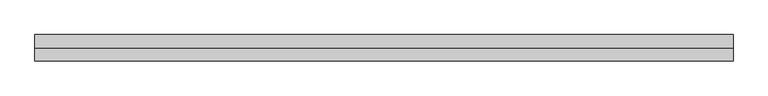
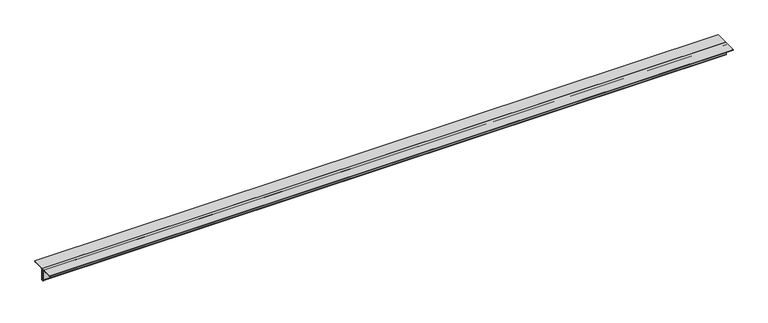
"""IFC4 building model written with IfcOpenShell, lengths in millimetres: member geometry, 0123_Steel Framing_2Ls-KSD3502 : H_SB_AR_S03_2Ls-130x130x12_HBR4."""

import ifcopenshell
import ifcopenshell.guid

model = None  # the IFC model being written
_history = None  # IfcOwnerHistory: only IFC2X3 demands one
_inside = {}  # id of a spatial element -> (the spatial element, [elements in it])
_under = {}  # id of a project, library or spatial element -> (it, [spatial elements below it])
_declared = {}  # id of a project -> (the project, [libraries it declares])
_typed = {}  # id of a type object -> (the type object, [elements of that type])
_made_of = {}  # id of a material, layer set ... -> (it, [elements and type objects made of it])


def new_model(schema):
    """Start an empty IFC model of exactly this schema.

    Asked for "IFC4X3", IfcOpenShell would pick the latest addendum, in which some entities
    have other attributes; the version numbers below select the first issue.
    IFC2X3 requires an IfcOwnerHistory on every rooted entity: one is made here for all.
    """
    global model, _history
    if schema == "IFC4X3":
        model = ifcopenshell.file(schema_version=(4, 3, 0, 0))
    else:
        model = ifcopenshell.file(schema=schema)
    _inside.clear()
    _under.clear()
    _declared.clear()
    _typed.clear()
    _made_of.clear()
    _history = None
    if model.schema == "IFC2X3":
        org = make("IfcOrganization", Name="unknown")
        user = make(
            "IfcPersonAndOrganization",
            ThePerson=make("IfcPerson", FamilyName="unknown"),
            TheOrganization=org,
        )
        app = make(
            "IfcApplication",
            ApplicationDeveloper=org,
            Version="unknown",
            ApplicationFullName="unknown",
            ApplicationIdentifier="unknown",
        )
        _history = make(
            "IfcOwnerHistory",
            OwningUser=user,
            OwningApplication=app,
            ChangeAction="ADDED",
            CreationDate=0,
        )
    return model


def make(cls, **values):
    """One entity of the class cls with the attributes given. An attribute that is None is left unset."""
    return model.create_entity(
        cls, **{name: value for name, value in values.items() if value is not None}
    )


def rooted(cls, **values):
    """An entity with a GlobalId (a new one), such as an element, a storey or a relation."""
    return make(cls, GlobalId=ifcopenshell.guid.new(), OwnerHistory=_history, **values)


def si_unit(unit_type, name, prefix=None):
    """IfcSIUnit, for example si_unit("LENGTHUNIT", "METRE", prefix="MILLI")."""
    return make("IfcSIUnit", UnitType=unit_type, Prefix=prefix, Name=name)


def assignment(units):
    """IfcUnitAssignment: the units of a project."""
    return None if units is None else make("IfcUnitAssignment", Units=units)


def point(xyz):
    """IfcCartesianPoint."""
    return None if xyz is None else make("IfcCartesianPoint", Coordinates=xyz)


def direction(xyz):
    """IfcDirection."""
    return None if xyz is None else make("IfcDirection", DirectionRatios=xyz)


def frame(location, z_axis=None, x_axis=None):
    """IfcAxis2Placement3D, a coordinate frame: its origin and axes. An axis left out is left unset."""
    return make(
        "IfcAxis2Placement3D",
        Location=point(location),
        Axis=direction(z_axis),
        RefDirection=direction(x_axis),
    )


def frame_2d(location, x_axis=None):
    """IfcAxis2Placement2D, a coordinate frame in the plane: its origin and x axis."""
    return make(
        "IfcAxis2Placement2D", Location=point(location), RefDirection=direction(x_axis)
    )


def origin():
    """The frame at (0, 0, 0) with its axes left unset."""
    return frame((0.0, 0.0, 0.0))


def place(relative_to, where):
    """IfcLocalPlacement: puts the frame where relative to a parent placement (None: the world)."""
    return make(
        "IfcLocalPlacement", PlacementRelTo=relative_to, RelativePlacement=where
    )


def context(
    kind, dimensions, precision=None, world=None, true_north=None, identifier=None
):
    """IfcGeometricRepresentationContext, for example the 3D "Model" context."""
    return make(
        "IfcGeometricRepresentationContext",
        ContextIdentifier=identifier,
        ContextType=kind,
        CoordinateSpaceDimension=dimensions,
        Precision=precision,
        WorldCoordinateSystem=world,
        TrueNorth=true_north,
    )


def project(units=None, contexts=None):
    """IfcProject with its units and contexts."""
    return rooted(
        "IfcProject",
        Name="project",
        RepresentationContexts=contexts,
        UnitsInContext=assignment(units),
    )


def spatial(cls, under=None, at=None, **own):
    """A site, building, storey or space (cls), placed at a placement, below another one or the project."""
    s = rooted(cls, ObjectPlacement=at, **own)
    if under is not None:
        _under.setdefault(under.id(), (under, []))[1].append(s)
    return s


def polyline(points):
    """IfcPolyline through the points."""
    return make("IfcPolyline", Points=[point(p) for p in points])


def circle_curve(where, radius):
    """IfcCircle in the frame where."""
    return make("IfcCircle", Position=where, Radius=radius)


def trimmed(basis, trim1, trim2, sense, master):
    """IfcTrimmedCurve: the piece of a basis curve between two trims."""
    return make(
        "IfcTrimmedCurve",
        BasisCurve=basis,
        Trim1=trim1,
        Trim2=trim2,
        SenseAgreement=sense,
        MasterRepresentation=master,
    )


def segment(curve, same_sense, transition):
    """IfcCompositeCurveSegment."""
    return make(
        "IfcCompositeCurveSegment",
        Transition=transition,
        SameSense=same_sense,
        ParentCurve=curve,
    )


def composite_curve(segments, self_intersect=None):
    """IfcCompositeCurve: segments joined end to end."""
    return make("IfcCompositeCurve", Segments=segments, SelfIntersect=self_intersect)


def outline(outer, holes=None, kind="AREA"):
    """IfcArbitraryClosedProfileDef: a profile drawn as a closed curve; with holes, ...WithVoids."""
    if holes is None:
        return make("IfcArbitraryClosedProfileDef", ProfileType=kind, OuterCurve=outer)
    return make(
        "IfcArbitraryProfileDefWithVoids",
        ProfileType=kind,
        OuterCurve=outer,
        InnerCurves=holes,
    )


def extrude(swept, where, along, depth):
    """IfcExtrudedAreaSolid: the profile swept, set in the frame where, extruded along a direction by depth."""
    return make(
        "IfcExtrudedAreaSolid",
        SweptArea=swept,
        Position=where,
        ExtrudedDirection=direction(along),
        Depth=depth,
    )


def shape(context_of_items, identifier, shape_type, items):
    """IfcShapeRepresentation: the items that make up one representation, for example the "Body"."""
    return make(
        "IfcShapeRepresentation",
        ContextOfItems=context_of_items,
        RepresentationIdentifier=identifier,
        RepresentationType=shape_type,
        Items=items,
    )


def source(mapping_origin, context_of_items, identifier, shape_type, items):
    """IfcRepresentationMap: a shape defined once, which mapped items show again and again."""
    return make(
        "IfcRepresentationMap",
        MappingOrigin=mapping_origin,
        MappedRepresentation=shape(context_of_items, identifier, shape_type, items),
    )


def transform(
    local_origin,
    x_axis=None,
    y_axis=None,
    z_axis=None,
    scale=None,
    scale2=None,
    scale3=None,
    uniform=True,
):
    """IfcCartesianTransformationOperator3D, or its non-uniform kind. x_axis, y_axis, z_axis: its Axis1, 2, 3."""
    if uniform:
        return make(
            "IfcCartesianTransformationOperator3D",
            Axis1=direction(x_axis),
            Axis2=direction(y_axis),
            LocalOrigin=point(local_origin),
            Scale=scale,
            Axis3=direction(z_axis),
        )
    return make(
        "IfcCartesianTransformationOperator3DnonUniform",
        Axis1=direction(x_axis),
        Axis2=direction(y_axis),
        LocalOrigin=point(local_origin),
        Scale=scale,
        Axis3=direction(z_axis),
        Scale2=scale2,
        Scale3=scale3,
    )


def mapped(mapping_source, mapping_target):
    """IfcMappedItem: shows the shape of a source again, moved by a transform."""
    return make(
        "IfcMappedItem", MappingSource=mapping_source, MappingTarget=mapping_target
    )


def made_of(thing, what):
    """Note that an element or type object is made of a material, layer set ...; save() writes the relation."""
    if what is not None:
        _made_of.setdefault(what.id(), (what, []))[1].append(thing)
    return thing


def element(
    cls,
    number,
    at=None,
    inside=None,
    cuts=None,
    type_object=None,
    material=None,
    context=None,
    identifier="Body",
    shape_type=None,
    held_by="IfcProductDefinitionShape",
    body=None,
    shapes=None,
    **own,
):
    """One element of the class cls, such as IfcWall. Its Tag is "e" and its number.

    at: its placement. inside: the storey or other place that contains it. cuts: it is an
    opening in that element (IfcRelVoidsElement). A single representation is given by context,
    identifier, shape_type and body (its items); several are given by shapes. held_by: the class
    of the entity that holds the representations. save() writes the other relations.
    """
    e = rooted(cls, Tag="e%d" % number, ObjectPlacement=at, **own)
    if body is not None:
        shapes = [shape(context, identifier, shape_type, body)]
    if shapes is not None:
        e.Representation = make(held_by, Representations=shapes)
    if inside is not None:
        _inside.setdefault(inside.id(), (inside, []))[1].append(e)
    if cuts is not None:
        rooted(
            "IfcRelVoidsElement", RelatingBuildingElement=cuts, RelatedOpeningElement=e
        )
    if type_object is not None:
        _typed.setdefault(type_object.id(), (type_object, []))[1].append(e)
    return made_of(e, material)


def aggregate(whole, parts):
    """IfcRelAggregates: a whole, such as a stair, and the parts it consists of."""
    return rooted("IfcRelAggregates", RelatingObject=whole, RelatedObjects=parts)


def save(model, path):
    """Write the relations noted so far, then the file.

    IfcRelAggregates (storeys below a building ...), IfcRelContainedInSpatialStructure (elements
    in a storey), IfcRelDefinesByType, IfcRelAssociatesMaterial and IfcRelDeclares: one each for
    every whole, place, type object, material and project.
    """
    for whole, parts in _under.values():
        aggregate(whole, parts)
    for where, things in _inside.values():
        rooted(
            "IfcRelContainedInSpatialStructure",
            RelatedElements=things,
            RelatingStructure=where,
        )
    for kind, things in _typed.values():
        rooted("IfcRelDefinesByType", RelatedObjects=things, RelatingType=kind)
    for what, things in _made_of.values():
        rooted("IfcRelAssociatesMaterial", RelatedObjects=things, RelatingMaterial=what)
    for by, libraries in _declared.values():
        rooted("IfcRelDeclares", RelatingContext=by, RelatedDefinitions=libraries)
    model.write(path)


def member_85476d18(model_context):
    return source(origin(), model_context, "Body", "SweptSolid", [
        extrude(outline(composite_curve([segment(polyline([(0.0, 36.4), (130.0, 36.4)]), True, "CONTINUOUS"), segment(trimmed(circle_curve(frame_2d((118.0, 36.4)), 12.0), [point((130.0, 36.4))], [point((118.0, 24.4))], False, "CARTESIAN"), True, "CONTINUOUS"), segment(polyline([(118.0, 24.4), (24.0, 24.4)]), True, "CONTINUOUS"), segment(trimmed(circle_curve(frame_2d((24.0, 12.4)), 12.0), [point((24.0, 24.4))], [point((12.0, 12.4))], True, "CARTESIAN"), True, "CONTINUOUS"), segment(polyline([(12.0, 12.4), (12.0, -81.6)]), True, "CONTINUOUS"), segment(trimmed(circle_curve(frame_2d((0.0, -81.6)), 12.0), [point((12.0, -81.6))], [point((0.0, -93.6))], False, "CARTESIAN"), True, "CONTINUOUS"), segment(polyline([(0.0, -93.6), (0.0, 36.4)]), True, "CONTINUOUS")], self_intersect=False)), frame((-3436.1943157, 0.0, 0.0), z_axis=(1.0, 0.0, 0.0), x_axis=(0.0, 1.0, 0.0)), (0.0, 0.0, 1.0), 6850.1941634),
        extrude(outline(composite_curve([segment(polyline([(0.0, 36.4), (0.0, -93.6)]), True, "CONTINUOUS"), segment(trimmed(circle_curve(frame_2d((0.0, -81.6)), 12.0), [point((0.0, -93.6))], [point((-12.0, -81.6))], False, "CARTESIAN"), True, "CONTINUOUS"), segment(polyline([(-12.0, -81.6), (-12.0, 12.4)]), True, "CONTINUOUS"), segment(trimmed(circle_curve(frame_2d((-24.0, 12.4)), 12.0), [point((-12.0, 12.4))], [point((-24.0, 24.4))], True, "CARTESIAN"), True, "CONTINUOUS"), segment(polyline([(-24.0, 24.4), (-118.0, 24.4)]), True, "CONTINUOUS"), segment(trimmed(circle_curve(frame_2d((-118.0, 36.4)), 12.0), [point((-118.0, 24.4))], [point((-130.0, 36.4))], False, "CARTESIAN"), True, "CONTINUOUS"), segment(polyline([(-130.0, 36.4), (0.0, 36.4)]), True, "CONTINUOUS")], self_intersect=False)), frame((-3436.1943157, 0.0, 0.0), z_axis=(1.0, 0.0, 0.0), x_axis=(0.0, 1.0, 0.0)), (0.0, 0.0, 1.0), 6850.1941634),
    ])


if __name__ == "__main__":
    model = new_model("IFC4")
    model_context = context("Model", 3, world=origin())
    ifc_project = project(units=[si_unit("LENGTHUNIT", "METRE", prefix="MILLI")], contexts=[model_context])
    site = spatial("IfcSite", under=ifc_project)
    building = spatial("IfcBuilding", under=site)
    placement = place(None, origin())
    member_shape = member_85476d18(model_context)
    element("IfcMember", 1, ObjectType="0123_Steel Framing_2Ls-KSD3502 : H_SB_AR_S03_2Ls-130x130x12_HBR4", at=placement, inside=building, context=model_context, shape_type="MappedRepresentation", body=[
        mapped(member_shape, transform((0.0, 0.0, 0.0), x_axis=(1.0, 0.0, 0.0), y_axis=(0.0, 1.0, 0.0), z_axis=(0.0, 0.0, 1.0))),
    ])
    save(model, "model.ifc")

# Revit data of these elements
# Type "0123_Steel Framing_2Ls-KSD3502 : H_SB_AR_S03_2Ls-130x130x12_HBR4"
#   Type Mark = "HBR4"
#   Assembly Code = "B10"
#   Legs = "SLBB"
#   W = 8.97
#   Perimeter = 1.04 m²/m
#   Nominal Weight = 46.80 kgf/m
#   Length [instance default] = 1000 mm
#   Space = 0 mm
#   b = 130 mm
#   d = 130 mm
#   t = 12 mm
#   y = 36.4 mm
#   A = 0.005952 m²
#   Structural Material [instance default] = Steel ASTM A36
# Element 1 (IfcMember, "0123_Steel Framing_2Ls-KSD3502 : H_SB_AR_S03_2Ls-130x130x12_HBR4")
#   Materials on its faces: "Steel ASTM A36"
# Materials
#   "Steel ASTM A36": class "Metal", colour RGB 199 199 199, transparency 0, Description = "Structural steel, ASTM A36 Grade B, mill finish", Cost = 0
